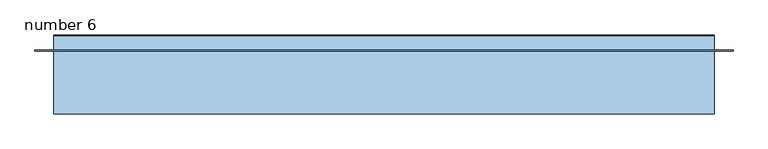
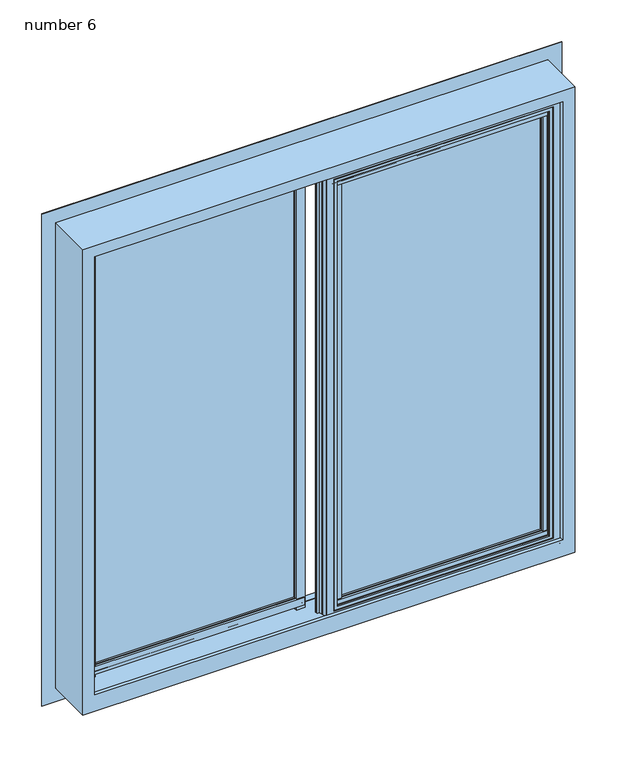
"""IFC4 building model written with IfcOpenShell, lengths in millimetres: window geometry, Window-Exterior-Sierra-Horizontal_Sliding_XO-36inch_Width-Standard : number 6."""

from ifc_helpers import new_model, si_unit, point, frame, frame_2d, origin, place, context, project, spatial, polyline, circle_curve, ellipse_curve, trimmed, segment, composite_curve, outline, extrude, faceted_brep, source, transform, mapped, element, save
from ifc_brep_helpers import plane_surface, cylinder_surface, revolved_surface, advanced_brep


def number_6_d5c00f89(model_context):
    return source(origin(), model_context, "Body", "SolidModel", [
        extrude(outline(polyline([(-30.95625, 959.3990662), (-42.06875, 960.3157287), (-42.06875, 980.7896808), (-30.95625, 981.7063433), (-30.95625, 959.3990662)])), frame((23.8125, 0.0, 0.0), z_axis=(1.0, 0.0, 0.0), x_axis=(0.0, 1.0, 0.0)), (0.0, 0.0, 1.0), 536.575),
        extrude(outline(polyline([(-11.90625, 981.7063433), (-0.6945312, 980.9337774), (-0.6945312, 960.1716321), (-11.90625, 959.3990662), (-11.90625, 981.7063433)])), frame((23.8125, 0.0, 0.0), z_axis=(1.0, 0.0, 0.0), x_axis=(0.0, 1.0, 0.0)), (0.0, 0.0, 1.0), 536.575),
        extrude(outline(composite_curve([segment(polyline([(-30.95625, 970.5465365), (-30.95625, 959.4453125), (-33.62325, 959.4453125), (-33.62325, 961.0201125)]), True, "CONTINUOUS"), segment(trimmed(circle_curve(frame_2d((-31.4860105, 966.253572)), 5.6530426), [point((-33.62325, 961.0201125))], [point((-37.12845, 966.5996458))], False, "CARTESIAN"), True, "CONTINUOUS"), segment(polyline([(-37.12845, 966.5996458), (-41.275, 966.5996458), (-41.275, 974.5159792), (-39.5097, 974.5159792)]), True, "CONTINUOUS"), segment(trimmed(circle_curve(frame_2d((-31.4860105, 974.862053)), 8.0311494), [point((-39.5097, 974.5159792))], [point((-37.5778298, 980.0955125))], False, "CARTESIAN"), True, "CONTINUOUS"), segment(polyline([(-37.5778298, 980.0955125), (-37.5778298, 981.6703125), (-30.95625, 981.6703125), (-30.95625, 970.5465365)]), True, "CONTINUOUS")], self_intersect=False)), frame((23.8125, 0.0, 0.0), z_axis=(1.0, 0.0, 0.0), x_axis=(0.0, 1.0, 0.0)), (0.0, 0.0, 1.0), 536.575),
        extrude(outline(polyline([(13.890625, 959.3990662), (2.778125, 960.3157287), (2.778125, 980.7896808), (13.890625, 981.7063433), (13.890625, 959.3990662)])), frame((-560.3875, 0.0, 0.0), z_axis=(1.0, 0.0, 0.0), x_axis=(0.0, 1.0, 0.0)), (0.0, 0.0, 1.0), 536.575),
        extrude(outline(polyline([(32.940625, 981.7063433), (44.1523438, 980.9337774), (44.1523438, 960.1716321), (32.940625, 959.3990662), (32.940625, 981.7063433)])), frame((-560.3875, 0.0, 0.0), z_axis=(1.0, 0.0, 0.0), x_axis=(0.0, 1.0, 0.0)), (0.0, 0.0, 1.0), 536.575),
        extrude(outline(composite_curve([segment(polyline([(13.890625, 970.5465365), (13.890625, 959.4453125), (11.223625, 959.4453125), (11.223625, 961.0201125)]), True, "CONTINUOUS"), segment(trimmed(circle_curve(frame_2d((13.3608645, 966.253572)), 5.6530426), [point((11.223625, 961.0201125))], [point((7.718425, 966.5996458))], False, "CARTESIAN"), True, "CONTINUOUS"), segment(polyline([(7.718425, 966.5996458), (3.571875, 966.5996458), (3.571875, 974.5159792), (5.337175, 974.5159792)]), True, "CONTINUOUS"), segment(trimmed(circle_curve(frame_2d((13.3608645, 974.862053)), 8.0311494), [point((5.337175, 974.5159792))], [point((7.2690452, 980.0955125))], False, "CARTESIAN"), True, "CONTINUOUS"), segment(polyline([(7.2690452, 980.0955125), (7.2690452, 981.6703125), (13.890625, 981.6703125), (13.890625, 970.5465365)]), True, "CONTINUOUS")], self_intersect=False)), frame((-560.3875, 0.0, 0.0), z_axis=(1.0, 0.0, 0.0), x_axis=(0.0, 1.0, 0.0)), (0.0, 0.0, 1.0), 536.575),
        extrude(outline(polyline([(13.890625, 2066.2834412), (2.778125, 2067.2001037), (2.778125, 2087.6740558), (13.890625, 2088.5907183), (13.890625, 2066.2834412)])), frame((-560.3875, 0.0, 0.0), z_axis=(1.0, 0.0, 0.0), x_axis=(0.0, 1.0, 0.0)), (0.0, 0.0, 1.0), 536.575),
        extrude(outline(polyline([(32.940625, 2088.5907183), (44.1523438, 2087.8181524), (44.1523438, 2067.0560071), (32.940625, 2066.2834412), (32.940625, 2088.5907183)])), frame((-560.3875, 0.0, 0.0), z_axis=(1.0, 0.0, 0.0), x_axis=(0.0, 1.0, 0.0)), (0.0, 0.0, 1.0), 536.575),
        extrude(outline(composite_curve([segment(polyline([(13.890625, 2077.4309115), (13.890625, 2066.3296875), (11.223625, 2066.3296875), (11.223625, 2067.9044875)]), True, "CONTINUOUS"), segment(trimmed(circle_curve(frame_2d((13.3608645, 2073.137947)), 5.6530426), [point((11.223625, 2067.9044875))], [point((7.718425, 2073.4840208))], False, "CARTESIAN"), True, "CONTINUOUS"), segment(polyline([(7.718425, 2073.4840208), (3.571875, 2073.4840208), (3.571875, 2081.4003542), (5.337175, 2081.4003542)]), True, "CONTINUOUS"), segment(trimmed(circle_curve(frame_2d((13.3608645, 2081.746428)), 8.0311494), [point((5.337175, 2081.4003542))], [point((7.2690452, 2086.9798875))], False, "CARTESIAN"), True, "CONTINUOUS"), segment(polyline([(7.2690452, 2086.9798875), (7.2690452, 2088.5546875), (13.890625, 2088.5546875), (13.890625, 2077.4309115)]), True, "CONTINUOUS")], self_intersect=False)), frame((-560.3875, 0.0, 0.0), z_axis=(1.0, 0.0, 0.0), x_axis=(0.0, 1.0, 0.0)), (0.0, 0.0, 1.0), 536.575),
        extrude(outline(polyline([(-30.95625, 2066.2834412), (-42.06875, 2067.2001037), (-42.06875, 2087.6740558), (-30.95625, 2088.5907183), (-30.95625, 2066.2834412)])), frame((23.8125, 0.0, 0.0), z_axis=(1.0, 0.0, 0.0), x_axis=(0.0, 1.0, 0.0)), (0.0, 0.0, 1.0), 536.575),
        extrude(outline(polyline([(-11.90625, 2088.5907183), (-0.6945312, 2087.8181524), (-0.6945312, 2067.0560071), (-11.90625, 2066.2834412), (-11.90625, 2088.5907183)])), frame((23.8125, 0.0, 0.0), z_axis=(1.0, 0.0, 0.0), x_axis=(0.0, 1.0, 0.0)), (0.0, 0.0, 1.0), 536.575),
        extrude(outline(composite_curve([segment(polyline([(-30.95625, 2077.4309115), (-30.95625, 2066.3296875), (-33.62325, 2066.3296875), (-33.62325, 2067.9044875)]), True, "CONTINUOUS"), segment(trimmed(circle_curve(frame_2d((-31.4860105, 2073.137947)), 5.6530426), [point((-33.62325, 2067.9044875))], [point((-37.12845, 2073.4840208))], False, "CARTESIAN"), True, "CONTINUOUS"), segment(polyline([(-37.12845, 2073.4840208), (-41.275, 2073.4840208), (-41.275, 2081.4003542), (-39.5097, 2081.4003542)]), True, "CONTINUOUS"), segment(trimmed(circle_curve(frame_2d((-31.4860105, 2081.746428)), 8.0311494), [point((-39.5097, 2081.4003542))], [point((-37.5778298, 2086.9798875))], False, "CARTESIAN"), True, "CONTINUOUS"), segment(polyline([(-37.5778298, 2086.9798875), (-37.5778298, 2088.5546875), (-30.95625, 2088.5546875), (-30.95625, 2077.4309115)]), True, "CONTINUOUS")], self_intersect=False)), frame((23.8125, 0.0, 0.0), z_axis=(1.0, 0.0, 0.0), x_axis=(0.0, 1.0, 0.0)), (0.0, 0.0, 1.0), 536.575),
        extrude(outline(polyline([(-563.0134338, 13.890625), (-540.7061567, 13.890625), (-541.6228192, 4.365625), (-562.0967713, 4.365625), (-563.0134338, 13.890625)])), frame((0.0, 0.0, 952.5), z_axis=(0.0, 0.0, 1.0), x_axis=(1.0, 0.0, 0.0)), (0.0, 0.0, 1.0), 1143.0),
        extrude(outline(polyline([(-540.7061567, 32.940625), (-563.0134338, 32.940625), (-562.2408679, 42.5648438), (-541.4787226, 42.5648438), (-540.7061567, 32.940625)])), frame((0.0, 0.0, 952.5), z_axis=(0.0, 0.0, 1.0), x_axis=(1.0, 0.0, 0.0)), (0.0, 0.0, 1.0), 1143.0),
        extrude(outline(composite_curve([segment(polyline([(-551.8659635, 13.890625), (-540.7421875, 13.890625), (-540.7421875, 9.5985242), (-542.3169875, 9.5985242)]), True, "CONTINUOUS"), segment(trimmed(circle_curve(frame_2d((-547.550447, 13.3608645)), 6.445487), [point((-542.3169875, 9.5985242))], [point((-547.8965208, 6.924675))], False, "CARTESIAN"), True, "CONTINUOUS"), segment(polyline([(-547.8965208, 6.924675), (-547.8965208, 5.159375), (-555.8128542, 5.159375), (-555.8128542, 7.718425)]), True, "CONTINUOUS"), segment(trimmed(circle_curve(frame_2d((-556.158928, 13.3608645)), 5.6530426), [point((-555.8128542, 7.718425))], [point((-561.3923875, 11.223625))], False, "CARTESIAN"), True, "CONTINUOUS"), segment(polyline([(-561.3923875, 11.223625), (-562.9671875, 11.223625), (-562.9671875, 13.890625), (-551.8659635, 13.890625)]), True, "CONTINUOUS")], self_intersect=False)), frame((0.0, 0.0, 952.5), z_axis=(0.0, 0.0, 1.0), x_axis=(1.0, 0.0, 0.0)), (0.0, 0.0, 1.0), 1143.0),
        extrude(outline(polyline([(563.0134338, -30.95625), (562.0967713, -40.48125), (541.6228192, -40.48125), (540.7061567, -30.95625), (563.0134338, -30.95625)])), frame((0.0, 0.0, 952.5), z_axis=(0.0, 0.0, 1.0), x_axis=(1.0, 0.0, 0.0)), (0.0, 0.0, 1.0), 1143.0),
        extrude(outline(polyline([(540.7061567, -11.90625), (541.4787226, -2.2820312), (562.2408679, -2.2820312), (563.0134338, -11.90625), (540.7061567, -11.90625)])), frame((0.0, 0.0, 952.5), z_axis=(0.0, 0.0, 1.0), x_axis=(1.0, 0.0, 0.0)), (0.0, 0.0, 1.0), 1143.0),
        extrude(outline(composite_curve([segment(polyline([(551.8659635, -30.95625), (562.9671875, -30.95625), (562.9671875, -33.62325), (561.3923875, -33.62325)]), True, "CONTINUOUS"), segment(trimmed(circle_curve(frame_2d((556.158928, -31.4860105)), 5.6530426), [point((561.3923875, -33.62325))], [point((555.8128542, -37.12845))], False, "CARTESIAN"), True, "CONTINUOUS"), segment(polyline([(555.8128542, -37.12845), (555.8128542, -39.6875), (547.8965208, -39.6875), (547.8965208, -37.9222)]), True, "CONTINUOUS"), segment(trimmed(circle_curve(frame_2d((547.550447, -31.4860105)), 6.445487), [point((547.8965208, -37.9222))], [point((542.3169875, -35.2483508))], False, "CARTESIAN"), True, "CONTINUOUS"), segment(polyline([(542.3169875, -35.2483508), (540.7421875, -35.2483508), (540.7421875, -30.95625), (551.8659635, -30.95625)]), True, "CONTINUOUS")], self_intersect=False)), frame((0.0, 0.0, 952.5), z_axis=(0.0, 0.0, 1.0), x_axis=(1.0, 0.0, 0.0)), (0.0, 0.0, 1.0), 1143.0),
        extrude(outline(polyline([(879.8514818, 644.1495838), (2168.1495838, 644.1495838), (2168.1495838, -644.1495838), (879.8514818, -644.1495838), (879.8514818, 644.1495838)]), holes=[polyline([(914.4200683, -609.5809972), (2133.5809972, -609.5809972), (2133.5809972, 609.5809972), (914.4200683, 609.5809972), (914.4200683, -609.5809972)])]), frame((0.0, 56.35625, 0.0), z_axis=(0.0, 1.0, 0.0), x_axis=(0.0, 0.0, 1.0)), (0.0, 0.0, 1.0), 1.3692925),
        faceted_brep([(592.2452673, 61.8007595, 2116.2452673), (594.5632068, 85.439324, 2118.5632068), (594.5632068, 85.439324, 915.510409), (592.2452673, 61.8007595, 915.510409), (-592.2452673, 61.8007595, 2116.2452673), (-594.5632068, 85.439324, 2118.5632068), (-609.6, -59.8487004, 2133.6), (609.6, -59.8487004, 2133.6), (609.6, 83.8857584, 2133.6), (-609.6, 83.8857584, 2133.6), (-592.2452673, 61.8007595, 915.510409), (-594.5632068, 85.439324, 915.510409), (580.1297286, -59.8487004, 2104.1297286), (580.1297286, -48.9537259, 2104.1297286), (580.1297286, -48.9537259, 950.6555073), (580.1297286, -50.9012589, 951.1326574), (580.1297286, -50.9012589, 957.3267373), (580.1297286, -59.8487004, 957.3267373), (592.6836, -48.9537259, 2116.6836), (592.6836, -1.4525069, 2116.6836), (592.6836, -1.4525069, 939.0175967), (592.6836, -48.9537259, 950.6555073), (583.5400777, -1.4525069, 2107.5400777), (583.5400777, 10.1171482, 2107.5400777), (583.5400777, 10.1171482, 936.1830039), (583.5400777, -1.4525069, 939.0175967), (578.4551976, 10.1171482, 2102.4551976), (578.4551976, 26.899095, 2102.4551976), (578.4551976, 26.899095, 932.0713873), (578.4551976, 10.1171482, 936.1830039), (-609.6, 83.8857584, 915.510409), (-609.6, 86.3576576, 915.510409), (-609.6, 86.3576576, 914.4), (-609.6, -59.8487004, 914.4), (609.6, -59.8487004, 914.4), (609.6, 86.3576576, 914.4), (609.6, 86.3576576, 915.510409), (609.6, 83.8857584, 915.510409), (-580.1297286, -59.8487004, 2104.1297286), (-580.1297286, -59.8487004, 957.3267373), (-580.1297286, -50.9012589, 957.3267373), (-580.1297286, -50.9012589, 951.1326574), (583.6170827, 26.899095, 932.0713873), (583.6170827, 39.894466, 928.8874908), (573.8057011, 41.2733658, 928.5496571), (573.2593437, 52.0255869, 925.9153376), (582.3829219, 52.0255869, 925.9153376), (582.3829219, 55.096925, 925.1628525), (577.977436, 55.096925, 925.1628525), (577.977436, 56.33085, 924.860538), (-577.977436, 56.3169605, 924.8639409), (-577.977436, 55.096925, 925.1628525), (-582.3829219, 55.096925, 925.1628525), (-582.3829219, 52.0255869, 925.9153376), (-573.2593437, 52.0255869, 925.9153376), (-573.8057011, 41.2733658, 928.5496571), (-583.6170827, 39.894466, 928.8874908), (-583.6170827, 26.899095, 932.0713873), (-578.4551976, 26.899095, 932.0713873), (-578.4551976, 10.1171482, 936.1830039), (-583.5400777, 10.1171482, 936.1830039), (-583.5400777, -1.4525069, 939.0175967), (-592.6836, -1.4525069, 939.0175967), (-592.6836, -48.9537259, 950.6555073), (-580.1297286, -48.9537259, 950.6555073), (577.977436, 57.6604904, 924.8639409), (-577.977436, 57.6604904, 924.8639409), (577.977436, 57.6604904, 915.510409), (-577.977436, 57.6604904, 915.510409), (-580.1297286, -48.9537259, 2104.1297286), (-592.6836, -48.9537259, 2116.6836), (-592.6836, -1.4525069, 2116.6836), (-583.5400777, -1.4525069, 2107.5400777), (-583.5400777, 10.1171482, 2107.5400777), (-578.4551976, 10.1171482, 2102.4551976), (-578.4551976, 26.899095, 2102.4551976), (-583.6170827, 26.899095, 2107.6170827), (583.6170827, 26.899095, 2107.6170827), (583.6170827, 39.894466, 2107.6170827), (573.8057011, 41.2733658, 2097.8057011), (-583.6170827, 39.894466, 2107.6170827), (-605.917, 85.439324, 915.510409), (-605.917, 85.439324, 2129.917), (605.917, 85.439324, 2129.917), (605.917, 85.439324, 915.510409), (605.917, 77.5357584, 2129.917), (605.917, 77.5357584, 915.510409), (-605.917, 77.5357584, 2129.917), (-605.917, 77.5357584, 915.510409), (-608.203, 77.5357584, 915.510409), (-608.203, 77.5357584, 2132.203), (608.203, 77.5357584, 2132.203), (608.203, 77.5357584, 915.510409), (608.203, 83.8857584, 2132.203), (608.203, 83.8857584, 915.510409), (-608.203, 83.8857584, 2132.203), (-608.203, 83.8857584, 915.510409), (-584.2071742, 61.8007595, 915.510409), (-584.2071742, 60.6800805, 915.510409), (-577.977436, 60.6800805, 915.510409), (577.977436, 60.6800805, 915.510409), (584.2071742, 60.6800805, 915.510409), (584.2071742, 61.8007595, 915.510409), (-573.8057011, 41.2733658, 2097.8057011), (573.2593437, 52.0255869, 2097.2593437), (-573.2593437, 52.0255869, 2097.2593437), (-582.3829219, 52.0255869, 2106.3829219), (582.3829219, 52.0255869, 2106.3829219), (582.3829219, 55.096925, 2106.3829219), (-582.3829219, 55.096925, 2106.3829219), (-577.977436, 55.096925, 2101.977436), (577.977436, 55.096925, 2101.977436), (577.977436, 60.6800805, 2101.977436), (-577.977436, 60.6800805, 2101.977436), (-584.2071742, 60.6800805, 2108.2071742), (584.2071742, 60.6800805, 2108.2071742), (584.2071742, 61.8007595, 2108.2071742), (-584.2071742, 61.8007595, 2108.2071742)], [[[0, 1, 2, 3]], [[1, 0, 4, 5]], [[6, 7, 8, 9]], [[5, 4, 10, 11]], [[12, 13, 14, 15, 16, 17]], [[18, 19, 20, 21]], [[22, 23, 24, 25]], [[26, 27, 28, 29]], [[6, 9, 30, 31, 32, 33]], [[8, 7, 34, 35, 36, 37]], [[35, 34, 33, 32]], [[7, 6, 33, 34], [38, 12, 17, 39]], [[39, 17, 16, 40]], [[40, 16, 15, 41]], [[41, 15, 14, 21, 20, 25, 24, 29, 28, 42, 43, 44, 45, 46, 47, 48, 49, 50, 51, 52, 53, 54, 55, 56, 57, 58, 59, 60, 61, 62, 63, 64]], [[65, 66, 50, 49]], [[66, 65, 67, 68]], [[13, 69, 64, 63, 70, 18, 21, 14]], [[19, 71, 62, 61, 72, 22, 25, 20]], [[23, 73, 60, 59, 74, 26, 29, 24]], [[27, 75, 58, 57, 76, 77, 42, 28]], [[77, 78, 43, 42]], [[78, 79, 44, 43]], [[12, 38, 69, 13]], [[18, 70, 71, 19]], [[22, 72, 73, 23]], [[26, 74, 75, 27]], [[77, 76, 80, 78]], [[69, 38, 39, 40, 41, 64]], [[71, 70, 63, 62]], [[73, 72, 61, 60]], [[75, 74, 59, 58]], [[80, 76, 57, 56]], [[1, 5, 11, 81, 82, 83, 84, 2]], [[83, 85, 86, 84]], [[85, 87, 88, 89, 90, 91, 92, 86]], [[91, 93, 94, 92]], [[9, 8, 37, 94, 93, 95, 96, 30]], [[83, 82, 87, 85]], [[91, 90, 95, 93]], [[87, 82, 81, 88]], [[95, 90, 89, 96]], [[36, 31, 30, 96, 89, 88, 81, 11, 10, 97, 98, 99, 68, 67, 100, 101, 102, 3, 2, 84, 86, 92, 94, 37]], [[32, 31, 36, 35]], [[79, 78, 80, 103]], [[103, 80, 56, 55]], [[79, 104, 45, 44]], [[104, 105, 54, 53, 106, 107, 46, 45]], [[107, 108, 47, 46]], [[108, 109, 52, 51, 110, 111, 48, 47]], [[111, 112, 100, 67, 65, 49, 48]], [[112, 113, 99, 98, 114, 115, 101, 100]], [[115, 116, 102, 101]], [[4, 0, 3, 102, 116, 117, 97, 10]], [[79, 103, 105, 104]], [[107, 106, 109, 108]], [[111, 110, 113, 112]], [[115, 114, 117, 116]], [[105, 103, 55, 54]], [[109, 106, 53, 52]], [[113, 110, 51, 50, 66, 68, 99]], [[117, 114, 98, 97]]]),
        extrude(outline(polyline([(43.5040588, -30.95625), (42.5873963, -40.48125), (22.1134442, -40.48125), (21.1967817, -30.95625), (43.5040588, -30.95625)])), frame((0.0, 0.0, 952.5), z_axis=(0.0, 0.0, 1.0), x_axis=(1.0, 0.0, 0.0)), (0.0, 0.0, 1.0), 1143.0),
        extrude(outline(polyline([(21.1967817, -11.90625), (21.9693476, -2.2820312), (42.7314929, -2.2820312), (43.5040588, -11.90625), (21.1967817, -11.90625)])), frame((0.0, 0.0, 952.5), z_axis=(0.0, 0.0, 1.0), x_axis=(1.0, 0.0, 0.0)), (0.0, 0.0, 1.0), 1143.0),
        extrude(outline(composite_curve([segment(polyline([(32.3565885, -30.95625), (43.4578125, -30.95625), (43.4578125, -33.62325), (41.8830125, -33.62325)]), True, "CONTINUOUS"), segment(trimmed(circle_curve(frame_2d((36.649553, -31.4860105)), 5.6530426), [point((41.8830125, -33.62325))], [point((36.3034792, -37.12845))], False, "CARTESIAN"), True, "CONTINUOUS"), segment(polyline([(36.3034792, -37.12845), (36.3034792, -39.6875), (28.3871458, -39.6875), (28.3871458, -37.9222)]), True, "CONTINUOUS"), segment(trimmed(circle_curve(frame_2d((28.041072, -31.4860105)), 6.445487), [point((28.3871458, -37.9222))], [point((22.8076125, -35.2483508))], False, "CARTESIAN"), True, "CONTINUOUS"), segment(polyline([(22.8076125, -35.2483508), (21.2328125, -35.2483508), (21.2328125, -30.95625), (32.3565885, -30.95625)]), True, "CONTINUOUS")], self_intersect=False)), frame((0.0, 0.0, 952.5), z_axis=(0.0, 0.0, 1.0), x_axis=(1.0, 0.0, 0.0)), (0.0, 0.0, 1.0), 1143.0),
        extrude(outline(polyline([(-43.5040588, 13.890625), (-21.1967817, 13.890625), (-22.1134442, 4.365625), (-42.5873963, 4.365625), (-43.5040588, 13.890625)])), frame((0.0, 0.0, 952.5), z_axis=(0.0, 0.0, 1.0), x_axis=(1.0, 0.0, 0.0)), (0.0, 0.0, 1.0), 1143.0),
        extrude(outline(polyline([(-21.1967817, 32.940625), (-43.5040588, 32.940625), (-42.7314929, 42.5648438), (-21.9693476, 42.5648438), (-21.1967817, 32.940625)])), frame((0.0, 0.0, 952.5), z_axis=(0.0, 0.0, 1.0), x_axis=(1.0, 0.0, 0.0)), (0.0, 0.0, 1.0), 1143.0),
        extrude(outline(composite_curve([segment(polyline([(-32.3565885, 13.890625), (-21.2328125, 13.890625), (-21.2328125, 9.5985242), (-22.8076125, 9.5985242)]), True, "CONTINUOUS"), segment(trimmed(circle_curve(frame_2d((-28.041072, 13.3608645)), 6.445487), [point((-22.8076125, 9.5985242))], [point((-28.3871458, 6.924675))], False, "CARTESIAN"), True, "CONTINUOUS"), segment(polyline([(-28.3871458, 6.924675), (-28.3871458, 5.159375), (-36.3034792, 5.159375), (-36.3034792, 7.718425)]), True, "CONTINUOUS"), segment(trimmed(circle_curve(frame_2d((-36.649553, 13.3608645)), 5.6530426), [point((-36.3034792, 7.718425))], [point((-41.8830125, 11.223625))], False, "CARTESIAN"), True, "CONTINUOUS"), segment(polyline([(-41.8830125, 11.223625), (-43.4578125, 11.223625), (-43.4578125, 13.890625), (-32.3565885, 13.890625)]), True, "CONTINUOUS")], self_intersect=False)), frame((0.0, 0.0, 952.5), z_axis=(0.0, 0.0, 1.0), x_axis=(1.0, 0.0, 0.0)), (0.0, 0.0, 1.0), 1143.0),
        extrude(outline(polyline([(563.75935, -11.90625), (563.75935, -30.955332), (20.44065, -30.955332), (20.44065, -11.90625), (563.75935, -11.90625)])), frame((0.0, 0.0, 958.65315), z_axis=(0.0, 0.0, 1.0), x_axis=(1.0, 0.0, 0.0)), (0.0, 0.0, 1.0), 1130.6937),
        advanced_brep(
        [(554.92015, -9.74725, 967.49235), (29.27985, -9.74725, 967.49235), (29.27985, -10.8831079, 967.49235), (554.92015, -10.8831079, 967.49235), (553.0833265, -7.3042106, 969.3291735), (31.1166735, -7.3042106, 969.3291735), (31.3062238, -9.74725, 969.5187238), (552.8937762, -9.74725, 969.5187238), (560.88915, -4.76885, 961.52335), (23.31085, -4.76885, 961.52335), (560.88915, -2.38125, 961.52335), (23.31085, -2.38125, 961.52335), (585.57795, -4.76885, 936.83455), (-1.37795, -4.76885, 936.83455), (1.00965, -2.38125, 939.22215), (583.19035, -2.38125, 939.22215), (585.57795, -7.33425, 936.83455), (-1.37795, -7.33425, 936.83455), (583.54595, -9.01065, 938.86655), (0.65405, -9.01065, 938.86655), (0.65405, -7.33425, 938.86655), (583.54595, -7.33425, 938.86655), (580.24395, -10.91565, 942.16855), (3.95605, -10.91565, 942.16855), (3.95605, -9.01065, 942.16855), (580.24395, -9.01065, 942.16855), (588.16875, -16.52905, 934.24375), (-3.96875, -16.52905, 934.24375), (-3.96875, -10.91565, 934.24375), (588.16875, -10.91565, 934.24375), (582.86015, -28.72105, 939.55235), (1.33985, -28.72105, 939.55235), (1.33985, -16.52905, 939.55235), (582.86015, -16.52905, 939.55235), (582.86015, -32.68345, 939.55235), (1.33985, -32.68345, 939.55235), (582.86015, -46.01845, 939.55235), (1.33985, -46.01845, 939.55235), (582.04735, -46.83125, 940.36515), (2.15265, -46.83125, 940.36515), (563.75935, -44.950732, 958.65315), (20.44065, -44.950732, 958.65315), (20.44065, -46.83125, 958.65315), (563.75935, -46.83125, 958.65315), (562.1584612, -46.550932, 960.2540388), (22.0415388, -46.550932, 960.2540388), (22.0415388, -44.950732, 960.2540388), (562.1584612, -44.950732, 960.2540388), (554.6146612, -42.7830125, 967.7978388), (29.5853388, -42.7830125, 967.7978388), (29.5853388, -46.550932, 967.7978388), (554.6146612, -46.550932, 967.7978388), (551.4396612, -30.955332, 970.9728388), (32.7603388, -30.955332, 970.9728388), (31.7476888, -42.7830125, 969.9601888), (552.4523112, -42.7830125, 969.9601888), (563.75935, -33.3436209, 958.65315), (20.44065, -33.3436209, 958.65315), (22.8289388, -30.955332, 961.0414388), (561.3710612, -30.955332, 961.0414388), (563.75935, -11.90625, 958.65315), (20.44065, -11.90625, 958.65315), (559.1555891, -10.8831079, 963.2569109), (25.0444109, -10.8831079, 963.2569109), (24.0212688, -11.90625, 962.2337688), (560.1787312, -11.90625, 962.2337688), (29.27985, -9.74725, 2080.50765), (29.27985, -10.8831079, 2080.50765), (31.1166735, -7.3042106, 2078.6708265), (31.3062238, -9.74725, 2078.4812762), (23.31085, -4.76885, 2086.47665), (23.31085, -2.38125, 2086.47665), (-1.37795, -4.76885, 2111.16545), (1.00965, -2.38125, 2108.77785), (-1.37795, -7.33425, 2111.16545), (0.65405, -9.01065, 2109.13345), (0.65405, -7.33425, 2109.13345), (3.95605, -10.91565, 2105.83145), (3.95605, -9.01065, 2105.83145), (-3.96875, -16.52905, 2113.75625), (-3.96875, -10.91565, 2113.75625), (1.33985, -28.72105, 2108.44765), (1.33985, -16.52905, 2108.44765), (1.33985, -32.68345, 2108.44765), (1.33985, -46.01845, 2108.44765), (2.15265, -46.83125, 2107.63485), (20.44065, -44.950732, 2089.34685), (20.44065, -46.83125, 2089.34685), (22.0415388, -46.550932, 2087.7459612), (22.0415388, -44.950732, 2087.7459612), (29.5853388, -42.7830125, 2080.2021612), (29.5853388, -46.550932, 2080.2021612), (32.7603388, -30.955332, 2077.0271612), (31.7476888, -42.7830125, 2078.0398112), (20.44065, -33.3436209, 2089.34685), (22.8289388, -30.955332, 2086.9585612), (20.44065, -11.90625, 2089.34685), (25.0444109, -10.8831079, 2084.7430891), (24.0212688, -11.90625, 2085.7662312), (554.92015, -9.74725, 2080.50765), (554.92015, -10.8831079, 2080.50765), (553.0833265, -7.3042106, 2078.6708265), (552.8937762, -9.74725, 2078.4812762), (560.88915, -4.76885, 2086.47665), (560.88915, -2.38125, 2086.47665), (585.57795, -4.76885, 2111.16545), (583.19035, -2.38125, 2108.77785), (585.57795, -7.33425, 2111.16545), (583.54595, -9.01065, 2109.13345), (583.54595, -7.33425, 2109.13345), (580.24395, -10.91565, 2105.83145), (580.24395, -9.01065, 2105.83145), (588.16875, -16.52905, 2113.75625), (588.16875, -10.91565, 2113.75625), (582.86015, -28.72105, 2108.44765), (582.86015, -16.52905, 2108.44765), (582.86015, -32.68345, 2108.44765), (582.86015, -46.01845, 2108.44765), (582.04735, -46.83125, 2107.63485), (563.75935, -44.950732, 2089.34685), (563.75935, -46.83125, 2089.34685), (562.1584612, -46.550932, 2087.7459612), (562.1584612, -44.950732, 2087.7459612), (554.6146612, -42.7830125, 2080.2021612), (554.6146612, -46.550932, 2080.2021612), (551.4396612, -30.955332, 2077.0271612), (552.4523112, -42.7830125, 2078.0398112), (563.75935, -33.3436209, 2089.34685), (561.3710612, -30.955332, 2086.9585612), (563.75935, -11.90625, 2089.34685), (559.1555891, -10.8831079, 2084.7430891), (560.1787312, -11.90625, 2085.7662312)],
        [
            (0, 1),
            (1, 2),
            (2, 3),
            (3, 0),
            (4, 5),
            (5, 6),
            (6, 7),
            (7, 4),
            (8, 9),
            (9, 5),
            (4, 8),
            (10, 11),
            (11, 9),
            (8, 10),
            (12, 13),
            (13, 14, ellipse_curve(frame((1.00965, -4.76885, 939.22215), z_axis=(0.7071067811865475, 0.0, -0.7071067811865475), x_axis=(0.7071067811865476, 0.0, 0.7071067811865474)), 3.3765763, 2.3876)),
            (14, 15),
            (15, 12, ellipse_curve(frame((583.19035, -4.76885, 939.22215), z_axis=(-0.7071067811865475, 0.0, -0.7071067811865475), x_axis=(0.7071067811865476, 0.0, -0.7071067811865474)), 3.3765763, 2.3876)),
            (16, 17),
            (17, 13),
            (12, 16),
            (18, 19),
            (19, 20),
            (20, 21),
            (21, 18),
            (22, 23),
            (23, 24),
            (24, 25),
            (25, 22),
            (26, 27),
            (27, 28),
            (28, 29),
            (29, 26),
            (30, 31),
            (31, 32),
            (32, 33),
            (33, 30),
            (34, 35),
            (35, 31, ellipse_curve(frame((1.33985, -30.70225, 939.55235), z_axis=(-0.7071067811865475, 0.0, 0.7071067811865475), x_axis=(-0.7071067811865476, 0.0, -0.7071067811865474)), 2.8018399, 1.9812)),
            (30, 34, ellipse_curve(frame((582.86015, -30.70225, 939.55235), z_axis=(0.7071067811865475, 0.0, 0.7071067811865475), x_axis=(-0.7071067811865476, 0.0, 0.7071067811865474)), 2.8018399, 1.9812)),
            (36, 37),
            (37, 35),
            (34, 36),
            (38, 39),
            (39, 37, ellipse_curve(frame((2.15265, -46.01845, 940.36515), z_axis=(0.7071067811865475, 0.0, -0.7071067811865475), x_axis=(0.7071067811865476, 0.0, 0.7071067811865474)), 1.1494728, 0.8128)),
            (36, 38, ellipse_curve(frame((582.04735, -46.01845, 940.36515), z_axis=(-0.7071067811865475, 0.0, -0.7071067811865475), x_axis=(0.7071067811865476, 0.0, -0.7071067811865474)), 1.1494728, 0.8128)),
            (40, 41),
            (41, 42),
            (42, 43),
            (43, 40),
            (44, 45),
            (45, 46),
            (46, 47),
            (47, 44),
            (48, 49),
            (49, 50),
            (50, 51),
            (51, 48),
            (52, 53),
            (53, 54),
            (54, 55),
            (55, 52),
            (56, 57),
            (57, 58),
            (58, 59),
            (59, 56),
            (60, 61),
            (61, 57),
            (56, 60),
            (62, 63),
            (63, 64),
            (64, 65),
            (65, 62),
            (1, 66),
            (66, 67),
            (67, 2),
            (5, 68),
            (68, 69),
            (69, 6),
            (9, 70),
            (70, 68),
            (11, 71),
            (71, 70),
            (13, 72),
            (72, 73, ellipse_curve(frame((1.00965, -4.76885, 2108.77785), z_axis=(-0.7071067811865475, 0.0, -0.7071067811865475), x_axis=(0.7071067811865474, 0.0, -0.7071067811865476)), 3.3765763, 2.3876)),
            (73, 14),
            (17, 74),
            (74, 72),
            (19, 75),
            (75, 76),
            (76, 20),
            (23, 77),
            (77, 78),
            (78, 24),
            (27, 79),
            (79, 80),
            (80, 28),
            (31, 81),
            (81, 82),
            (82, 32),
            (35, 83),
            (83, 81, ellipse_curve(frame((1.33985, -30.70225, 2108.44765), z_axis=(0.7071067811865475, 0.0, 0.7071067811865475), x_axis=(-0.7071067811865474, 0.0, 0.7071067811865476)), 2.8018399, 1.9812)),
            (37, 84),
            (84, 83),
            (39, 85),
            (85, 84, ellipse_curve(frame((2.15265, -46.01845, 2107.63485), z_axis=(-0.7071067811865475, 0.0, -0.7071067811865475), x_axis=(0.7071067811865474, 0.0, -0.7071067811865476)), 1.1494728, 0.8128)),
            (41, 86),
            (86, 87),
            (87, 42),
            (45, 88),
            (88, 89),
            (89, 46),
            (49, 90),
            (90, 91),
            (91, 50),
            (53, 92),
            (92, 93),
            (93, 54),
            (57, 94),
            (94, 95),
            (95, 58),
            (61, 96),
            (96, 94),
            (63, 97),
            (97, 98),
            (98, 64),
            (66, 99),
            (99, 100),
            (100, 67),
            (68, 101),
            (101, 102),
            (102, 69),
            (70, 103),
            (103, 101),
            (71, 104),
            (104, 103),
            (72, 105),
            (105, 106, ellipse_curve(frame((583.19035, -4.76885, 2108.77785), z_axis=(-0.7071067811865475, 0.0, 0.7071067811865475), x_axis=(-0.7071067811865476, 0.0, -0.7071067811865474)), 3.3765763, 2.3876)),
            (106, 73),
            (74, 107),
            (107, 105),
            (75, 108),
            (108, 109),
            (109, 76),
            (77, 110),
            (110, 111),
            (111, 78),
            (79, 112),
            (112, 113),
            (113, 80),
            (81, 114),
            (114, 115),
            (115, 82),
            (83, 116),
            (116, 114, ellipse_curve(frame((582.86015, -30.70225, 2108.44765), z_axis=(0.7071067811865475, 0.0, -0.7071067811865475), x_axis=(0.7071067811865476, 0.0, 0.7071067811865474)), 2.8018399, 1.9812)),
            (84, 117),
            (117, 116),
            (85, 118),
            (118, 117, ellipse_curve(frame((582.04735, -46.01845, 2107.63485), z_axis=(-0.7071067811865475, 0.0, 0.7071067811865475), x_axis=(-0.7071067811865476, 0.0, -0.7071067811865474)), 1.1494728, 0.8128)),
            (86, 119),
            (119, 120),
            (120, 87),
            (88, 121),
            (121, 122),
            (122, 89),
            (90, 123),
            (123, 124),
            (124, 91),
            (92, 125),
            (125, 126),
            (126, 93),
            (94, 127),
            (127, 128),
            (128, 95),
            (96, 129),
            (129, 127),
            (97, 130),
            (130, 131),
            (131, 98),
            (62, 130),
            (100, 3),
            (99, 0),
            (102, 7),
            (101, 4),
            (103, 8),
            (104, 10),
            (106, 15),
            (105, 12),
            (107, 16),
            (109, 21),
            (108, 18),
            (111, 25),
            (110, 22),
            (113, 29),
            (112, 26),
            (115, 33),
            (114, 30),
            (116, 34),
            (117, 36),
            (118, 38),
            (120, 43),
            (119, 40),
            (122, 47),
            (121, 44),
            (124, 51),
            (123, 48),
            (126, 55),
            (125, 52),
            (128, 59),
            (127, 56),
            (129, 60),
            (131, 65),
        ],
        [
            plane_surface(frame((554.92015, -10.8831079, 967.49235), z_axis=(0.0, 0.0, 1.0), x_axis=(-1.0, 0.0, 0.0))),
            plane_surface(frame((552.8937762, -9.74725, 969.5187238), z_axis=(0.0, 0.07735544009934268, 0.9970035786731345), x_axis=(-1.0, 0.0, 0.0))),
            plane_surface(frame((553.0833265, -7.3042106, 969.3291735), z_axis=(0.0, 0.9510889261909005, 0.3089172291683326), x_axis=(-1.0, 0.0, 0.0))),
            plane_surface(frame((560.88915, -4.76885, 961.52335), z_axis=(0.0, 0.0, 1.0), x_axis=(-1.0, 0.0, 0.0))),
            cylinder_surface(frame((588.16875, -4.76885, 939.22215), z_axis=(1.0, 0.0, 0.0), x_axis=(0.0, -1.0, 0.0)), 2.3876),
            plane_surface(frame((585.57795, -4.76885, 936.83455), z_axis=(0.0, 0.0, -1.0), x_axis=(-1.0, 0.0, 0.0))),
            plane_surface(frame((583.54595, -7.33425, 938.86655), z_axis=(0.0, 0.0, -1.0), x_axis=(-1.0, 0.0, 0.0))),
            plane_surface(frame((580.24395, -9.01065, 942.16855), z_axis=(0.0, 0.0, -1.0), x_axis=(-1.0, 0.0, 0.0))),
            plane_surface(frame((588.16875, -10.91565, 934.24375), z_axis=(0.0, 0.0, -1.0), x_axis=(-1.0, 0.0, 0.0))),
            plane_surface(frame((582.86015, -16.52905, 939.55235), z_axis=(0.0, 0.0, -1.0), x_axis=(-1.0, 0.0, 0.0))),
            revolved_surface(polyline([(-0.6413499930890794, -32.68345, 939.55235), (584.841349993089, -32.68345, 939.55235)]), (588.16875, -30.70225, 939.55235), (-1.0, 0.0, 0.0)),
            plane_surface(frame((582.86015, -32.68345, 939.55235), z_axis=(0.0, 0.0, -1.0), x_axis=(-1.0, 0.0, 0.0))),
            cylinder_surface(frame((588.16875, -46.01845, 940.36515), z_axis=(1.0, 0.0, 0.0), x_axis=(0.0, -1.0, 0.0)), 0.8128),
            plane_surface(frame((563.75935, -46.83125, 958.65315), z_axis=(0.0, 0.0, 1.0), x_axis=(-1.0, 0.0, 0.0))),
            plane_surface(frame((562.1584612, -44.950732, 960.2540388), z_axis=(0.0, 0.0, -1.0), x_axis=(-1.0, 0.0, 0.0))),
            plane_surface(frame((554.6146612, -46.550932, 967.7978388), z_axis=(0.0, 0.0, 1.0), x_axis=(-1.0, 0.0, 0.0))),
            plane_surface(frame((552.4523112, -42.7830125, 969.9601888), z_axis=(0.0, -0.08530487454184647, 0.996354895797376), x_axis=(-1.0, 0.0, 0.0))),
            plane_surface(frame((561.3710612, -30.955332, 961.0414388), z_axis=(0.0, 0.7071067811865713, -0.7071067811865238), x_axis=(-1.0, 0.0, 0.0))),
            plane_surface(frame((563.75935, -33.3436209, 958.65315), z_axis=(0.0, 0.0, 1.0), x_axis=(-1.0, 0.0, 0.0))),
            plane_surface(frame((560.1787312, -11.90625, 962.2337688), z_axis=(0.0, -0.7071067811861558, 0.7071067811869393), x_axis=(-1.0, 0.0, 0.0))),
            plane_surface(frame((29.27985, -10.8831079, 967.49235), z_axis=(1.0, 0.0, 0.0), x_axis=(0.0, 0.0, 1.0))),
            plane_surface(frame((31.3062238, -9.74725, 969.5187238), z_axis=(0.9970035786731345, 0.07735544009934263, 0.0), x_axis=(0.0, 0.0, 1.0))),
            plane_surface(frame((31.1166735, -7.3042106, 969.3291735), z_axis=(0.30891722916833264, 0.9510889261909005, 0.0), x_axis=(0.0, 0.0, 1.0))),
            plane_surface(frame((23.31085, -4.76885, 961.52335), z_axis=(1.0, 0.0, 0.0), x_axis=(0.0, 0.0, 1.0))),
            cylinder_surface(frame((1.00965, -4.76885, 934.24375), z_axis=(0.0, 0.0, -1.0), x_axis=(0.0, -1.0, 0.0)), 2.3876),
            plane_surface(frame((-1.37795, -4.76885, 936.83455), z_axis=(-1.0, 0.0, 0.0), x_axis=(0.0, 0.0, 1.0))),
            plane_surface(frame((0.65405, -7.33425, 938.86655), z_axis=(-1.0, 0.0, 0.0), x_axis=(0.0, 0.0, 1.0))),
            plane_surface(frame((3.95605, -9.01065, 942.16855), z_axis=(-1.0, 0.0, 0.0), x_axis=(0.0, 0.0, 1.0))),
            plane_surface(frame((-3.96875, -10.91565, 934.24375), z_axis=(-1.0, 0.0, 0.0), x_axis=(0.0, 0.0, 1.0))),
            plane_surface(frame((1.33985, -16.52905, 939.55235), z_axis=(-1.0, 0.0, 0.0), x_axis=(0.0, 0.0, 1.0))),
            revolved_surface(polyline([(1.33985, -32.68345, 2110.428849993089), (1.33985, -32.68345, 937.571150006911)]), (1.33985, -30.70225, 934.24375), (0.0, 0.0, 1.0)),
            plane_surface(frame((1.33985, -32.68345, 939.55235), z_axis=(-1.0, 0.0, 0.0), x_axis=(0.0, 0.0, 1.0))),
            cylinder_surface(frame((2.15265, -46.01845, 934.24375), z_axis=(0.0, 0.0, -1.0), x_axis=(0.0, -1.0, 0.0)), 0.8128),
            plane_surface(frame((20.44065, -46.83125, 958.65315), z_axis=(1.0, 0.0, 0.0), x_axis=(0.0, 0.0, 1.0))),
            plane_surface(frame((22.0415388, -44.950732, 960.2540388), z_axis=(-1.0, 0.0, 0.0), x_axis=(0.0, 0.0, 1.0))),
            plane_surface(frame((29.5853388, -46.550932, 967.7978388), z_axis=(1.0, 0.0, 0.0), x_axis=(0.0, 0.0, 1.0))),
            plane_surface(frame((31.7476888, -42.7830125, 969.9601888), z_axis=(0.996354895797376, -0.08530487454184653, 0.0), x_axis=(0.0, 0.0, 1.0))),
            plane_surface(frame((22.8289388, -30.955332, 961.0414388), z_axis=(-0.7071067811865238, 0.7071067811865713, 0.0), x_axis=(0.0, 0.0, 1.0))),
            plane_surface(frame((20.44065, -33.3436209, 958.65315), z_axis=(1.0, 0.0, 0.0), x_axis=(0.0, 0.0, 1.0))),
            plane_surface(frame((24.0212688, -11.90625, 962.2337688), z_axis=(0.7071067811869393, -0.7071067811861558, 0.0), x_axis=(0.0, 0.0, 1.0))),
            plane_surface(frame((29.27985, -10.8831079, 2080.50765), z_axis=(0.0, 0.0, -1.0), x_axis=(1.0, 0.0, 0.0))),
            plane_surface(frame((31.3062238, -9.74725, 2078.4812762), z_axis=(0.0, 0.07735544009934257, -0.9970035786731345), x_axis=(1.0, 0.0, 0.0))),
            plane_surface(frame((31.1166735, -7.3042106, 2078.6708265), z_axis=(0.0, 0.9510889261909005, -0.3089172291683327), x_axis=(1.0, 0.0, 0.0))),
            plane_surface(frame((23.31085, -4.76885, 2086.47665), z_axis=(0.0, 0.0, -1.0), x_axis=(1.0, 0.0, 0.0))),
            cylinder_surface(frame((-3.96875, -4.76885, 2108.77785), z_axis=(-1.0, 0.0, 0.0), x_axis=(0.0, -1.0, 0.0)), 2.3876),
            plane_surface(frame((-1.37795, -4.76885, 2111.16545), z_axis=(0.0, 0.0, 1.0), x_axis=(1.0, 0.0, 0.0))),
            plane_surface(frame((0.65405, -7.33425, 2109.13345), z_axis=(0.0, 0.0, 1.0), x_axis=(1.0, 0.0, 0.0))),
            plane_surface(frame((3.95605, -9.01065, 2105.83145), z_axis=(0.0, 0.0, 1.0), x_axis=(1.0, 0.0, 0.0))),
            plane_surface(frame((-3.96875, -10.91565, 2113.75625), z_axis=(0.0, 0.0, 1.0), x_axis=(1.0, 0.0, 0.0))),
            plane_surface(frame((1.33985, -16.52905, 2108.44765), z_axis=(0.0, 0.0, 1.0), x_axis=(1.0, 0.0, 0.0))),
            revolved_surface(polyline([(584.841349993089, -32.68345, 2108.44765), (-0.6413499930890376, -32.68345, 2108.44765)]), (-3.96875, -30.70225, 2108.44765), (1.0, 0.0, 0.0)),
            plane_surface(frame((1.33985, -32.68345, 2108.44765), z_axis=(0.0, 0.0, 1.0), x_axis=(1.0, 0.0, 0.0))),
            cylinder_surface(frame((-3.96875, -46.01845, 2107.63485), z_axis=(-1.0, 0.0, 0.0), x_axis=(0.0, -1.0, 0.0)), 0.8128),
            plane_surface(frame((20.44065, -46.83125, 2089.34685), z_axis=(0.0, 0.0, -1.0), x_axis=(1.0, 0.0, 0.0))),
            plane_surface(frame((22.0415388, -44.950732, 2087.7459612), z_axis=(0.0, 0.0, 1.0), x_axis=(1.0, 0.0, 0.0))),
            plane_surface(frame((29.5853388, -46.550932, 2080.2021612), z_axis=(0.0, 0.0, -1.0), x_axis=(1.0, 0.0, 0.0))),
            plane_surface(frame((31.7476888, -42.7830125, 2078.0398112), z_axis=(0.0, -0.08530487454184658, -0.996354895797376), x_axis=(1.0, 0.0, 0.0))),
            plane_surface(frame((22.8289388, -30.955332, 2086.9585612), z_axis=(0.0, 0.7071067811865713, 0.7071067811865238), x_axis=(1.0, 0.0, 0.0))),
            plane_surface(frame((20.44065, -33.3436209, 2089.34685), z_axis=(0.0, 0.0, -1.0), x_axis=(1.0, 0.0, 0.0))),
            plane_surface(frame((24.0212688, -11.90625, 2085.7662312), z_axis=(0.0, -0.7071067811861558, -0.7071067811869393), x_axis=(1.0, 0.0, 0.0))),
            plane_surface(frame((559.1555891, -10.8831079, 2084.7430891), z_axis=(0.0, -1.0, 0.0), x_axis=(0.0, 0.0, -1.0))),
            plane_surface(frame((554.92015, -10.8831079, 2080.50765), z_axis=(-1.0, 0.0, 0.0), x_axis=(0.0, 0.0, -1.0))),
            plane_surface(frame((554.92015, -9.74725, 2080.50765), z_axis=(0.0, -1.0, 0.0), x_axis=(0.0, 0.0, -1.0))),
            plane_surface(frame((552.8937762, -9.74725, 2078.4812762), z_axis=(-0.9970035786731345, 0.07735544009934263, 0.0), x_axis=(0.0, 0.0, -1.0))),
            plane_surface(frame((553.0833265, -7.3042106, 2078.6708265), z_axis=(-0.30891722916833264, 0.9510889261909005, 0.0), x_axis=(0.0, 0.0, -1.0))),
            plane_surface(frame((560.88915, -4.76885, 2086.47665), z_axis=(-1.0, 0.0, 0.0), x_axis=(0.0, 0.0, -1.0))),
            plane_surface(frame((560.88915, -2.38125, 2086.47665), z_axis=(0.0, 1.0, 0.0), x_axis=(0.0, 0.0, -1.0))),
            cylinder_surface(frame((583.19035, -4.76885, 2113.75625), z_axis=(0.0, 0.0, 1.0), x_axis=(0.0, -1.0, 0.0)), 2.3876),
            plane_surface(frame((585.57795, -4.76885, 2111.16545), z_axis=(1.0, 0.0, 0.0), x_axis=(0.0, 0.0, -1.0))),
            plane_surface(frame((585.57795, -7.33425, 2111.16545), z_axis=(0.0, -1.0, 0.0), x_axis=(0.0, 0.0, -1.0))),
            plane_surface(frame((583.54595, -7.33425, 2109.13345), z_axis=(1.0, 0.0, 0.0), x_axis=(0.0, 0.0, -1.0))),
            plane_surface(frame((583.54595, -9.01065, 2109.13345), z_axis=(0.0, -1.0, 0.0), x_axis=(0.0, 0.0, -1.0))),
            plane_surface(frame((580.24395, -9.01065, 2105.83145), z_axis=(1.0, 0.0, 0.0), x_axis=(0.0, 0.0, -1.0))),
            plane_surface(frame((580.24395, -10.91565, 2105.83145), z_axis=(0.0, 1.0, 0.0), x_axis=(0.0, 0.0, -1.0))),
            plane_surface(frame((588.16875, -10.91565, 2113.75625), z_axis=(1.0, 0.0, 0.0), x_axis=(0.0, 0.0, -1.0))),
            plane_surface(frame((588.16875, -16.52905, 2113.75625), z_axis=(0.0, -1.0, 0.0), x_axis=(0.0, 0.0, -1.0))),
            plane_surface(frame((582.86015, -16.52905, 2108.44765), z_axis=(1.0, 0.0, 0.0), x_axis=(0.0, 0.0, -1.0))),
            revolved_surface(polyline([(582.86015, -32.68345, 937.5711500069108), (582.86015, -32.68345, 2110.428849993089)]), (582.86015, -30.70225, 2113.75625), (0.0, 0.0, -1.0)),
            plane_surface(frame((582.86015, -32.68345, 2108.44765), z_axis=(1.0, 0.0, 0.0), x_axis=(0.0, 0.0, -1.0))),
            cylinder_surface(frame((582.04735, -46.01845, 2113.75625), z_axis=(0.0, 0.0, 1.0), x_axis=(0.0, -1.0, 0.0)), 0.8128),
            plane_surface(frame((582.04735, -46.83125, 2107.63485), z_axis=(0.0, -1.0, 0.0), x_axis=(0.0, 0.0, -1.0))),
            plane_surface(frame((563.75935, -46.83125, 2089.34685), z_axis=(-1.0, 0.0, 0.0), x_axis=(0.0, 0.0, -1.0))),
            plane_surface(frame((563.75935, -44.950732, 2089.34685), z_axis=(0.0, -1.0, 0.0), x_axis=(0.0, 0.0, -1.0))),
            plane_surface(frame((562.1584612, -44.950732, 2087.7459612), z_axis=(1.0, 0.0, 0.0), x_axis=(0.0, 0.0, -1.0))),
            plane_surface(frame((562.1584612, -46.550932, 2087.7459612), z_axis=(0.0, -1.0, 0.0), x_axis=(0.0, 0.0, -1.0))),
            plane_surface(frame((554.6146612, -46.550932, 2080.2021612), z_axis=(-1.0, 0.0, 0.0), x_axis=(0.0, 0.0, -1.0))),
            plane_surface(frame((554.6146612, -42.7830125, 2080.2021612), z_axis=(0.0, -1.0, 0.0), x_axis=(0.0, 0.0, -1.0))),
            plane_surface(frame((552.4523112, -42.7830125, 2078.0398112), z_axis=(-0.996354895797376, -0.08530487454184653, 0.0), x_axis=(0.0, 0.0, -1.0))),
            plane_surface(frame((551.4396612, -30.955332, 2077.0271612), z_axis=(0.0, 1.0, 0.0), x_axis=(0.0, 0.0, -1.0))),
            plane_surface(frame((561.3710612, -30.955332, 2086.9585612), z_axis=(0.7071067811865238, 0.7071067811865713, 0.0), x_axis=(0.0, 0.0, -1.0))),
            plane_surface(frame((563.75935, -33.3436209, 2089.34685), z_axis=(-1.0, 0.0, 0.0), x_axis=(0.0, 0.0, -1.0))),
            plane_surface(frame((563.75935, -11.90625, 2089.34685), z_axis=(0.0, -1.0, 0.0), x_axis=(0.0, 0.0, -1.0))),
            plane_surface(frame((560.1787312, -11.90625, 2085.7662312), z_axis=(-0.7071067811869393, -0.7071067811861558, 0.0), x_axis=(0.0, 0.0, -1.0))),
        ],
        [
            (0, [[1, 2, 3, 4]]),
            (1, [[5, 6, 7, 8]]),
            (2, [[9, 10, -5, 11]]),
            (3, [[12, 13, -9, 14]]),
            (4, [[15, 16, 17, 18]]),
            (5, [[19, 20, -15, 21]]),
            (6, [[22, 23, 24, 25]]),
            (7, [[26, 27, 28, 29]]),
            (8, [[30, 31, 32, 33]]),
            (9, [[34, 35, 36, 37]]),
            (10, [[38, 39, -34, 40]]),
            (11, [[41, 42, -38, 43]]),
            (12, [[44, 45, -41, 46]]),
            (13, [[47, 48, 49, 50]]),
            (14, [[51, 52, 53, 54]]),
            (15, [[55, 56, 57, 58]]),
            (16, [[59, 60, 61, 62]]),
            (17, [[63, 64, 65, 66]]),
            (18, [[67, 68, -63, 69]]),
            (19, [[70, 71, 72, 73]]),
            (20, [[74, 75, 76, -2]]),
            (21, [[77, 78, 79, -6]]),
            (22, [[80, 81, -77, -10]]),
            (23, [[82, 83, -80, -13]]),
            (24, [[84, 85, 86, -16]]),
            (25, [[87, 88, -84, -20]]),
            (26, [[89, 90, 91, -23]]),
            (27, [[92, 93, 94, -27]]),
            (28, [[95, 96, 97, -31]]),
            (29, [[98, 99, 100, -35]]),
            (30, [[101, 102, -98, -39]]),
            (31, [[103, 104, -101, -42]]),
            (32, [[105, 106, -103, -45]]),
            (33, [[107, 108, 109, -48]]),
            (34, [[110, 111, 112, -52]]),
            (35, [[113, 114, 115, -56]]),
            (36, [[116, 117, 118, -60]]),
            (37, [[119, 120, 121, -64]]),
            (38, [[122, 123, -119, -68]]),
            (39, [[124, 125, 126, -71]]),
            (40, [[127, 128, 129, -75]]),
            (41, [[130, 131, 132, -78]]),
            (42, [[133, 134, -130, -81]]),
            (43, [[135, 136, -133, -83]]),
            (44, [[137, 138, 139, -85]]),
            (45, [[140, 141, -137, -88]]),
            (46, [[142, 143, 144, -90]]),
            (47, [[145, 146, 147, -93]]),
            (48, [[148, 149, 150, -96]]),
            (49, [[151, 152, 153, -99]]),
            (50, [[154, 155, -151, -102]]),
            (51, [[156, 157, -154, -104]]),
            (52, [[158, 159, -156, -106]]),
            (53, [[160, 161, 162, -108]]),
            (54, [[163, 164, 165, -111]]),
            (55, [[166, 167, 168, -114]]),
            (56, [[169, 170, 171, -117]]),
            (57, [[172, 173, 174, -120]]),
            (58, [[175, 176, -172, -123]]),
            (59, [[177, 178, 179, -125]]),
            (60, [[-70, 180, -177, -124], [-3, -76, -129, 181]]),
            (61, [[182, -4, -181, -128]]),
            (62, [[-1, -182, -127, -74], [-7, -79, -132, 183]]),
            (63, [[184, -8, -183, -131]]),
            (64, [[185, -11, -184, -134]]),
            (65, [[186, -14, -185, -136]]),
            (66, [[-17, -86, -139, 187], [-12, -186, -135, -82]]),
            (67, [[188, -18, -187, -138]]),
            (68, [[189, -21, -188, -141]]),
            (69, [[-19, -189, -140, -87], [-24, -91, -144, 190]]),
            (70, [[191, -25, -190, -143]]),
            (71, [[-22, -191, -142, -89], [-28, -94, -147, 192]]),
            (72, [[193, -29, -192, -146]]),
            (73, [[-32, -97, -150, 194], [-26, -193, -145, -92]]),
            (74, [[195, -33, -194, -149]]),
            (75, [[-30, -195, -148, -95], [-36, -100, -153, 196]]),
            (76, [[197, -37, -196, -152]]),
            (77, [[198, -40, -197, -155]]),
            (78, [[199, -43, -198, -157]]),
            (79, [[200, -46, -199, -159]]),
            (80, [[-44, -200, -158, -105], [-49, -109, -162, 201]]),
            (81, [[202, -50, -201, -161]]),
            (82, [[-47, -202, -160, -107], [-53, -112, -165, 203]]),
            (83, [[204, -54, -203, -164]]),
            (84, [[-51, -204, -163, -110], [-57, -115, -168, 205]]),
            (85, [[206, -58, -205, -167]]),
            (86, [[-55, -206, -166, -113], [-61, -118, -171, 207]]),
            (87, [[208, -62, -207, -170]]),
            (88, [[-65, -121, -174, 209], [-59, -208, -169, -116]]),
            (89, [[210, -66, -209, -173]]),
            (90, [[211, -69, -210, -176]]),
            (91, [[-67, -211, -175, -122], [-72, -126, -179, 212]]),
            (92, [[-180, -73, -212, -178]]),
        ],
    ),
        extrude(outline(polyline([(-563.75935, 32.940625), (-20.44065, 32.940625), (-20.44065, 13.891543), (-563.75935, 13.891543), (-563.75935, 32.940625)])), frame((0.0, 0.0, 958.65315), z_axis=(0.0, 0.0, 1.0), x_axis=(1.0, 0.0, 0.0)), (0.0, 0.0, 1.0), 1130.6937),
    ])


if __name__ == "__main__":
    model = new_model("IFC4")
    model_context = context("Model", 3, world=origin())
    ifc_project = project(units=[si_unit("LENGTHUNIT", "METRE", prefix="MILLI")], contexts=[model_context])
    site = spatial("IfcSite", under=ifc_project)
    building = spatial("IfcBuilding", under=site)
    placement = place(None, origin())
    number_6_shape = number_6_d5c00f89(model_context)
    element("IfcWindow", 1, ObjectType="Window-Exterior-Sierra-Horizontal_Sliding_XO-36inch_Width-Standard : number 6", at=placement, inside=building, context=model_context, shape_type="MappedRepresentation", body=[
        mapped(number_6_shape, transform((0.0, 0.0, 0.0), x_axis=(1.0, 0.0, 0.0), y_axis=(0.0, 1.0, 0.0), z_axis=(0.0, 0.0, 1.0))),
    ])
    save(model, "model.ifc")

# Revit data of these elements
# Type "Window-Exterior-Sierra-Horizontal_Sliding_XO-36inch_Width-Standard : number 6"
#   Type Mark = "54"
#   URL = "http://www.sierrapacificwindows.com"
#   Triple Glaze Note = "Triple glazed options with respective limits"
#   Simulite Note = "Custom Simulite Options Available"
#   Product data url = "https://bimobject.com/sierrapacificwindows/product/sierrapacificwindows_horizontal-sliding-windows"
#   Product Page URL = "http://www.sierrapacificwindows.com/horizontal-sliding-windows.cfm"
#   Product Documentation Link = "http://www.sierrapacificwindows.com/architectural/drawings/pdfs/c-ws_13.pdf"
#   Model = "C-WS-3648"
#   Manufacturer = "Sierra Pacific Windows"
#   Jamb Extension Note = "Extension Jamb may be applied on some applications. Contact your SPW sales rep. for more information"
#   Glass Type = "Insulated Glass"
#   Description = "Energy efficient, durable, and secure window"
#   Construction Type = "Wood/Clad"
#   Assembly Code = "B2030230"
#   Window Pane Thickness = 0' - 0 3/4"
#   Vertical Simulite Length = 3' - 9"
#   Thickness = 0' - 1 3/4"
#   Simulite Wood Thickness Vertical = 0' - 0 11/32"
#   Simulite Wood Thickness Horizontal = 0' - 0 13/32"
#   Simulite Width = 0' - 0 7/8"
#   Simulite Clad Thickness Vertical = 0' - 0 11/32"
#   Simulite Clad Thickness Horizontal = 0' - 0 13/32"
#   Setback = 0' - 0"
#   Rough Width = 5' - 0 3/4"
#   Rough Height = 4' - 0 3/4"
#   Quarter Window Width = 1' - 0 1/2"
#   Interior Setback = 0' - 0"
#   Horizontal Simulite Length = 1' - 9 1/8"
#   Half Frame Width = 2' - 0 7/8"
#   Frame Width = 5' - 0"
#   Height = 4' - 0"
#   Width = 5' - 0"
#   Frame Height = 4' - 0"
#   First Simulite Width = 1' - 8 7/16"
#   First Simulite Height = 3' - 7 9/16"
#   Default Sill Height = 3' - 0"
#   Actual Width = 4' - 0"
#   Actual Height = 4' - 0"
#   Actual Half Width = 2' - 0"
#   Actual Glass Width = 1' - 8 7/16"
#   Actual Glass Height = 3' - 7 9/16"
#   Total Number of Lites Per Panel = 1
#   Simulites Visibility = yes
#   Number of Vertical Simulites Greater than One = 2
#   Number of Vertical Lites Per Panel = 1
#   Number of Horizontal Simulites Greater than One = 2
#   Number of Horizontal Lites Per Panel = 1
#   Vertical Simulite Type = element 483283
#   Interior Simulite = Wood - Sierra Pacific - Pine
#   Interior Panel Material = Wood - Sierra Pacific - Pine
#   Horizontal Simulite Type = element 483288
#   Glass = Glass - Sierra Doors - Clear
#   Frame = douglas fir
#   Exterior Simulite = Paint - Sierra Pacific - White 001
#   Exterior Panel Material = Paint - Sierra Pacific - White 001
#   Wall Closure = (empty or 0)
# Element 1 (IfcWindow, "Window-Exterior-Sierra-Horizontal_Sliding_XO-36inch_Width-Standard : number 6")
#   Materials on its faces: "Wood - Sierra Pacific - Pine", "Paint - Sierra Pacific - White 001", "douglas fir", "Glass - Sierra Doors - Clear"
# Materials
#   "Wood - Sierra Pacific - Pine": class "Miscellaneous", colour RGB 136 105 68, transparency 0
#   "Glass - Sierra Doors - Clear": class "Glass", colour RGB 0 0 255, transparency 0.75
#   "douglas fir": class "Generic", colour RGB 120 120 120, transparency 0, Cost = 0
#   "Paint - Sierra Pacific - White 001": class "Miscellaneous", colour RGB 111 112 111, transparency 0
